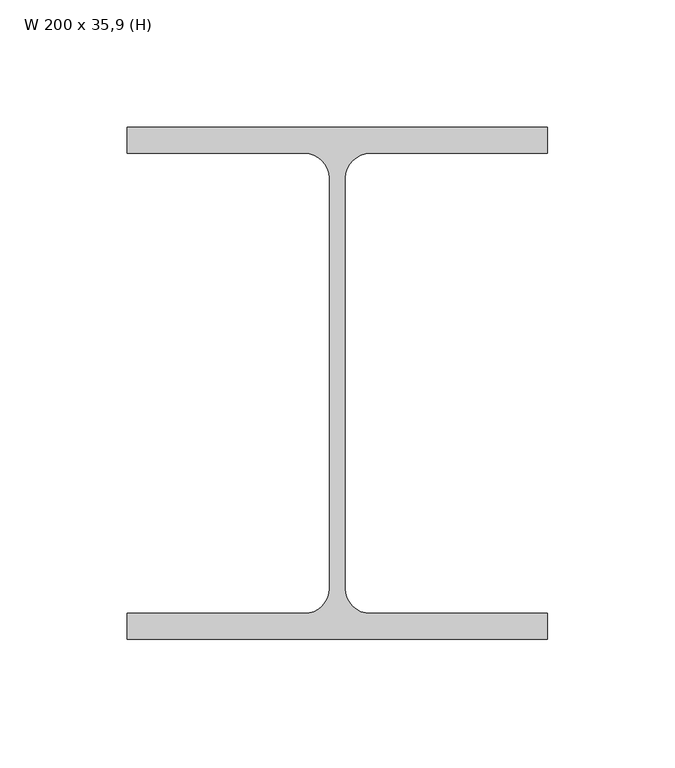
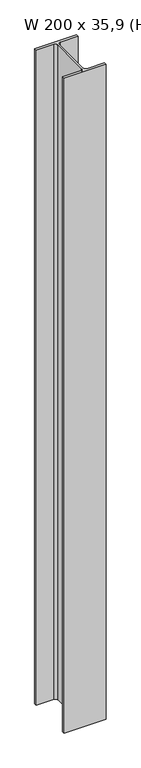
"""IFC4 building model written with IfcOpenShell, lengths in millimetres: column geometry, Pilar de Aço - H : W 200 x 35,9 (H)."""

from ifc_helpers import new_model, si_unit, point, frame_2d, origin, origin_with_axes, place, context, project, spatial, polyline, circle_curve, trimmed, segment, composite_curve, outline, extrude, source, transform, mapped, element, save


def w_200_x_35_9_h_b15f7e58(model_context):
    return source(origin(), model_context, "Body", "SweptSolid", [
        extrude(outline(composite_curve([segment(polyline([(82.5, 100.5), (82.5, 90.3), (12.9, 90.3)]), True, "CONTINUOUS"), segment(trimmed(circle_curve(frame_2d((12.9, 80.5)), 9.8), [point((12.9, 90.3))], [point((3.1, 80.5))], True, "CARTESIAN"), True, "CONTINUOUS"), segment(polyline([(3.1, 80.5), (3.1, -80.5)]), True, "CONTINUOUS"), segment(trimmed(circle_curve(frame_2d((12.9, -80.5)), 9.8), [point((3.1, -80.5))], [point((12.9, -90.3))], True, "CARTESIAN"), True, "CONTINUOUS"), segment(polyline([(12.9, -90.3), (82.5, -90.3), (82.5, -100.5), (-82.5, -100.5), (-82.5, -90.3), (-12.9, -90.3)]), True, "CONTINUOUS"), segment(trimmed(circle_curve(frame_2d((-12.9, -80.5)), 9.8), [point((-12.9, -90.3))], [point((-3.1, -80.5))], True, "CARTESIAN"), True, "CONTINUOUS"), segment(polyline([(-3.1, -80.5), (-3.1, 80.5)]), True, "CONTINUOUS"), segment(trimmed(circle_curve(frame_2d((-12.9, 80.5)), 9.8), [point((-3.1, 80.5))], [point((-12.9, 90.3))], True, "CARTESIAN"), True, "CONTINUOUS"), segment(polyline([(-12.9, 90.3), (-82.5, 90.3), (-82.5, 100.5), (82.5, 100.5)]), True, "CONTINUOUS")], self_intersect=False)), origin_with_axes(), (0.0, 0.0, 1.0), 2720.0),
    ])


if __name__ == "__main__":
    model = new_model("IFC4")
    model_context = context("Model", 3, world=origin())
    ifc_project = project(units=[si_unit("LENGTHUNIT", "METRE", prefix="MILLI")], contexts=[model_context])
    site = spatial("IfcSite", under=ifc_project)
    building = spatial("IfcBuilding", under=site)
    placement = place(None, origin())
    w_200_x_35_9_h_shape = w_200_x_35_9_h_b15f7e58(model_context)
    element("IfcColumn", 1, ObjectType="Pilar de Aço - H : W 200 x 35,9 (H)", at=placement, inside=building, context=model_context, shape_type="MappedRepresentation", body=[
        mapped(w_200_x_35_9_h_shape, transform((0.0, 0.0, 0.0), x_axis=(1.0, 0.0, 0.0), y_axis=(0.0, 1.0, 0.0), z_axis=(0.0, 0.0, 1.0))),
    ])
    save(model, "model.ifc")

# Revit data of these elements
# Type "Pilar de Aço - H : W 200 x 35,9 (H)"
#   SINAPI = ""
#   Área da seção = 45.7 m²
#   tw = 0.62 cm
#   tf = 1.02 cm
#   h = 18.06 cm
#   d' = 16.10 cm
#   d = 20.10 cm
#   bf = 16.50 cm
#   R = 0.98 cm
#   Massa Linear kg/m = 35.9
#   Aço = Metal - Aço 345MPa
#   Assembly Code = ""
# Materials
#   "Metal - Aço 345MPa": class "Metal", colour RGB 189 187 185, transparency 0, Cost = 0
